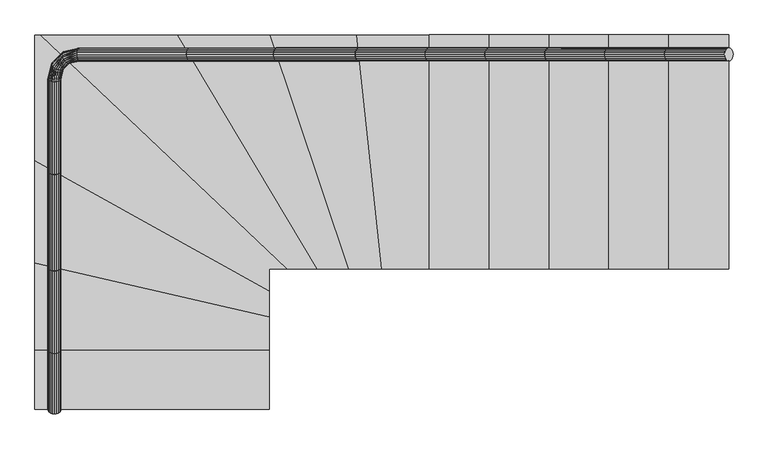
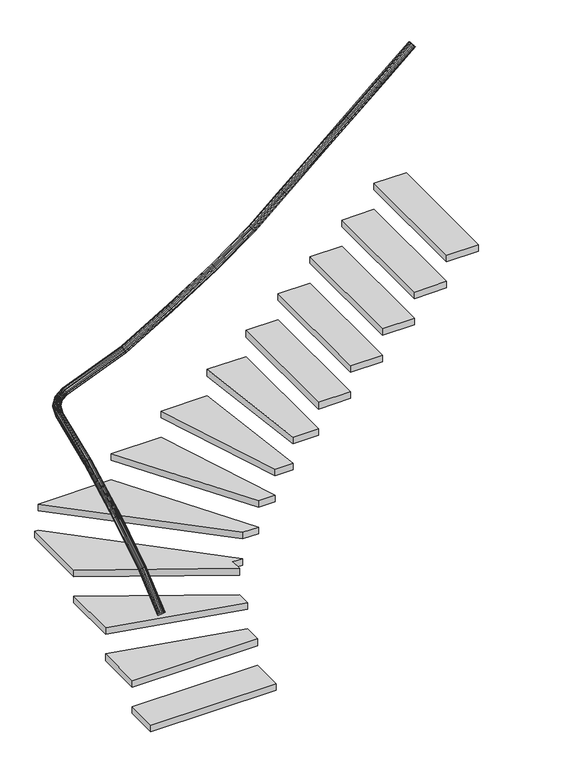
"""IFC4 building model written with IfcOpenShell, lengths in millimetres: stair geometry, 0_3d_modell."""

import ifcopenshell
import ifcopenshell.guid

model = None  # the IFC model being written
_history = None  # IfcOwnerHistory: only IFC2X3 demands one
_inside = {}  # id of a spatial element -> (the spatial element, [elements in it])
_under = {}  # id of a project, library or spatial element -> (it, [spatial elements below it])
_declared = {}  # id of a project -> (the project, [libraries it declares])
_typed = {}  # id of a type object -> (the type object, [elements of that type])
_made_of = {}  # id of a material, layer set ... -> (it, [elements and type objects made of it])


def new_model(schema):
    """Start an empty IFC model of exactly this schema.

    Asked for "IFC4X3", IfcOpenShell would pick the latest addendum, in which some entities
    have other attributes; the version numbers below select the first issue.
    IFC2X3 requires an IfcOwnerHistory on every rooted entity: one is made here for all.
    """
    global model, _history
    if schema == "IFC4X3":
        model = ifcopenshell.file(schema_version=(4, 3, 0, 0))
    else:
        model = ifcopenshell.file(schema=schema)
    _inside.clear()
    _under.clear()
    _declared.clear()
    _typed.clear()
    _made_of.clear()
    _history = None
    if model.schema == "IFC2X3":
        org = make("IfcOrganization", Name="unknown")
        user = make(
            "IfcPersonAndOrganization",
            ThePerson=make("IfcPerson", FamilyName="unknown"),
            TheOrganization=org,
        )
        app = make(
            "IfcApplication",
            ApplicationDeveloper=org,
            Version="unknown",
            ApplicationFullName="unknown",
            ApplicationIdentifier="unknown",
        )
        _history = make(
            "IfcOwnerHistory",
            OwningUser=user,
            OwningApplication=app,
            ChangeAction="ADDED",
            CreationDate=0,
        )
    return model


def make(cls, **values):
    """One entity of the class cls with the attributes given. An attribute that is None is left unset."""
    return model.create_entity(
        cls, **{name: value for name, value in values.items() if value is not None}
    )


def rooted(cls, **values):
    """An entity with a GlobalId (a new one), such as an element, a storey or a relation."""
    return make(cls, GlobalId=ifcopenshell.guid.new(), OwnerHistory=_history, **values)


def si_unit(unit_type, name, prefix=None):
    """IfcSIUnit, for example si_unit("LENGTHUNIT", "METRE", prefix="MILLI")."""
    return make("IfcSIUnit", UnitType=unit_type, Prefix=prefix, Name=name)


def assignment(units):
    """IfcUnitAssignment: the units of a project."""
    return None if units is None else make("IfcUnitAssignment", Units=units)


def point(xyz):
    """IfcCartesianPoint."""
    return None if xyz is None else make("IfcCartesianPoint", Coordinates=xyz)


def direction(xyz):
    """IfcDirection."""
    return None if xyz is None else make("IfcDirection", DirectionRatios=xyz)


def frame(location, z_axis=None, x_axis=None):
    """IfcAxis2Placement3D, a coordinate frame: its origin and axes. An axis left out is left unset."""
    return make(
        "IfcAxis2Placement3D",
        Location=point(location),
        Axis=direction(z_axis),
        RefDirection=direction(x_axis),
    )


def origin():
    """The frame at (0, 0, 0) with its axes left unset."""
    return frame((0.0, 0.0, 0.0))


def origin_with_axes():
    """The frame at (0, 0, 0) with the z axis (0, 0, 1) and the x axis (1, 0, 0) written out."""
    return frame((0.0, 0.0, 0.0), z_axis=(0.0, 0.0, 1.0), x_axis=(1.0, 0.0, 0.0))


def place(relative_to, where):
    """IfcLocalPlacement: puts the frame where relative to a parent placement (None: the world)."""
    return make(
        "IfcLocalPlacement", PlacementRelTo=relative_to, RelativePlacement=where
    )


def context(
    kind, dimensions, precision=None, world=None, true_north=None, identifier=None
):
    """IfcGeometricRepresentationContext, for example the 3D "Model" context."""
    return make(
        "IfcGeometricRepresentationContext",
        ContextIdentifier=identifier,
        ContextType=kind,
        CoordinateSpaceDimension=dimensions,
        Precision=precision,
        WorldCoordinateSystem=world,
        TrueNorth=true_north,
    )


def project(units=None, contexts=None):
    """IfcProject with its units and contexts."""
    return rooted(
        "IfcProject",
        Name="project",
        RepresentationContexts=contexts,
        UnitsInContext=assignment(units),
    )


def spatial(cls, under=None, at=None, **own):
    """A site, building, storey or space (cls), placed at a placement, below another one or the project."""
    s = rooted(cls, ObjectPlacement=at, **own)
    if under is not None:
        _under.setdefault(under.id(), (under, []))[1].append(s)
    return s


def polyline(points):
    """IfcPolyline through the points."""
    return make("IfcPolyline", Points=[point(p) for p in points])


def outline(outer, holes=None, kind="AREA"):
    """IfcArbitraryClosedProfileDef: a profile drawn as a closed curve; with holes, ...WithVoids."""
    if holes is None:
        return make("IfcArbitraryClosedProfileDef", ProfileType=kind, OuterCurve=outer)
    return make(
        "IfcArbitraryProfileDefWithVoids",
        ProfileType=kind,
        OuterCurve=outer,
        InnerCurves=holes,
    )


def extrude(swept, where, along, depth):
    """IfcExtrudedAreaSolid: the profile swept, set in the frame where, extruded along a direction by depth."""
    return make(
        "IfcExtrudedAreaSolid",
        SweptArea=swept,
        Position=where,
        ExtrudedDirection=direction(along),
        Depth=depth,
    )


def faces_of(points, faces, orient=None, outer=None):
    """IfcFace entities. A face is a list of loops; a loop is a list of indices into points, from 0.

    orient and outer hold one flag for each loop. By default every Orientation is true, the
    first loop of a face is its IfcFaceOuterBound and the others are IfcFaceBound.
    """
    made = []
    for i, loops in enumerate(faces):
        bounds = []
        for j, loop in enumerate(loops):
            is_outer = j == 0 if outer is None else outer[i][j]
            bounds.append(
                make(
                    "IfcFaceOuterBound" if is_outer else "IfcFaceBound",
                    Bound=make("IfcPolyLoop", Polygon=[points[k] for k in loop]),
                    Orientation=True if orient is None else orient[i][j],
                )
            )
        made.append(make("IfcFace", Bounds=bounds))
    return made


def faceted_brep(points, faces, orient=None, outer=None, voids=None):
    """IfcFacetedBrep: a solid bounded by flat faces; with voids (closed shells), ...WithVoids."""
    shared = [point(p) for p in points]
    hull = make("IfcClosedShell", CfsFaces=faces_of(shared, faces, orient, outer))
    if voids is None:
        return make("IfcFacetedBrep", Outer=hull)
    return make(
        "IfcFacetedBrepWithVoids",
        Outer=hull,
        Voids=[
            make(cls, CfsFaces=faces_of(shared, fs, o, b)) for cls, fs, o, b in voids
        ],
    )


def shape(context_of_items, identifier, shape_type, items):
    """IfcShapeRepresentation: the items that make up one representation, for example the "Body"."""
    return make(
        "IfcShapeRepresentation",
        ContextOfItems=context_of_items,
        RepresentationIdentifier=identifier,
        RepresentationType=shape_type,
        Items=items,
    )


def source(mapping_origin, context_of_items, identifier, shape_type, items):
    """IfcRepresentationMap: a shape defined once, which mapped items show again and again."""
    return make(
        "IfcRepresentationMap",
        MappingOrigin=mapping_origin,
        MappedRepresentation=shape(context_of_items, identifier, shape_type, items),
    )


def transform(
    local_origin,
    x_axis=None,
    y_axis=None,
    z_axis=None,
    scale=None,
    scale2=None,
    scale3=None,
    uniform=True,
):
    """IfcCartesianTransformationOperator3D, or its non-uniform kind. x_axis, y_axis, z_axis: its Axis1, 2, 3."""
    if uniform:
        return make(
            "IfcCartesianTransformationOperator3D",
            Axis1=direction(x_axis),
            Axis2=direction(y_axis),
            LocalOrigin=point(local_origin),
            Scale=scale,
            Axis3=direction(z_axis),
        )
    return make(
        "IfcCartesianTransformationOperator3DnonUniform",
        Axis1=direction(x_axis),
        Axis2=direction(y_axis),
        LocalOrigin=point(local_origin),
        Scale=scale,
        Axis3=direction(z_axis),
        Scale2=scale2,
        Scale3=scale3,
    )


def mapped(mapping_source, mapping_target):
    """IfcMappedItem: shows the shape of a source again, moved by a transform."""
    return make(
        "IfcMappedItem", MappingSource=mapping_source, MappingTarget=mapping_target
    )


def made_of(thing, what):
    """Note that an element or type object is made of a material, layer set ...; save() writes the relation."""
    if what is not None:
        _made_of.setdefault(what.id(), (what, []))[1].append(thing)
    return thing


def element(
    cls,
    number,
    at=None,
    inside=None,
    cuts=None,
    type_object=None,
    material=None,
    context=None,
    identifier="Body",
    shape_type=None,
    held_by="IfcProductDefinitionShape",
    body=None,
    shapes=None,
    **own,
):
    """One element of the class cls, such as IfcWall. Its Tag is "e" and its number.

    at: its placement. inside: the storey or other place that contains it. cuts: it is an
    opening in that element (IfcRelVoidsElement). A single representation is given by context,
    identifier, shape_type and body (its items); several are given by shapes. held_by: the class
    of the entity that holds the representations. save() writes the other relations.
    """
    e = rooted(cls, Tag="e%d" % number, ObjectPlacement=at, **own)
    if body is not None:
        shapes = [shape(context, identifier, shape_type, body)]
    if shapes is not None:
        e.Representation = make(held_by, Representations=shapes)
    if inside is not None:
        _inside.setdefault(inside.id(), (inside, []))[1].append(e)
    if cuts is not None:
        rooted(
            "IfcRelVoidsElement", RelatingBuildingElement=cuts, RelatedOpeningElement=e
        )
    if type_object is not None:
        _typed.setdefault(type_object.id(), (type_object, []))[1].append(e)
    return made_of(e, material)


def aggregate(whole, parts):
    """IfcRelAggregates: a whole, such as a stair, and the parts it consists of."""
    return rooted("IfcRelAggregates", RelatingObject=whole, RelatedObjects=parts)


def save(model, path):
    """Write the relations noted so far, then the file.

    IfcRelAggregates (storeys below a building ...), IfcRelContainedInSpatialStructure (elements
    in a storey), IfcRelDefinesByType, IfcRelAssociatesMaterial and IfcRelDeclares: one each for
    every whole, place, type object, material and project.
    """
    for whole, parts in _under.values():
        aggregate(whole, parts)
    for where, things in _inside.values():
        rooted(
            "IfcRelContainedInSpatialStructure",
            RelatedElements=things,
            RelatingStructure=where,
        )
    for kind, things in _typed.values():
        rooted("IfcRelDefinesByType", RelatedObjects=things, RelatingType=kind)
    for what, things in _made_of.values():
        rooted("IfcRelAssociatesMaterial", RelatedObjects=things, RelatingMaterial=what)
    for by, libraries in _declared.values():
        rooted("IfcRelDeclares", RelatingContext=by, RelatedDefinitions=libraries)
    model.write(path)


def stair_7a128c32(model_context):
    return source(origin(), model_context, "Body", "SolidModel", [
        faceted_brep([(51.2235871, 11.6788974, 875.6088541), (50.0, 16.9018591, 869.5592366), (51.2235871, 22.1248208, 863.5096191), (54.7745751, 26.8365226, 858.0521803), (60.3053687, 30.5757504, 853.7211323), (67.2745751, 32.9764824, 850.9404284), (75.0, 33.8037182, 849.9822631), (82.7254249, 32.9764824, 850.9404284), (89.6946313, 30.5757504, 853.7211323), (95.2254249, 26.8365226, 858.0521803), (98.7764129, 22.1248208, 863.5096191), (100.0, 16.9018591, 869.5592366), (98.7764129, 11.6788974, 875.6088541), (95.2254249, 6.9671956, 881.0662929), (89.6946313, 3.2279679, 885.3973409), (82.7254249, 0.8272359, 888.1780448), (75.0, 0.0, 889.1362101), (67.2745751, 0.8272359, 888.1780448), (60.3053687, 3.2279679, 885.3973409), (54.7745751, 6.9671956, 881.0662929), (51.2235871, 251.6675536, 1061.6862641), (50.0, 246.9018591, 1068.1306652), (51.2235871, 242.1361647, 1074.5750662), (54.7745751, 237.8369696, 1080.3886444), (60.3053687, 234.4251091, 1085.0023262), (67.2745751, 232.2345598, 1087.9644922), (75.0, 231.4797479, 1088.985185), (82.7254249, 232.2345598, 1087.9644922), (89.6946313, 234.4251091, 1085.0023262), (95.2254249, 237.8369696, 1080.3886444), (98.7764129, 242.1361647, 1074.5750662), (100.0, 246.9018591, 1068.1306652), (98.7764129, 251.6675536, 1061.6862641), (95.2254249, 255.9667486, 1055.872686), (89.6946313, 259.3786091, 1051.2590042), (82.7254249, 261.5691584, 1048.2968382), (75.0, 262.3239703, 1047.2761453), (67.2745751, 261.5691584, 1048.2968382), (60.3053687, 259.3786091, 1051.2590042), (54.7745751, 255.9667486, 1055.872686)], [[[0, 1, 2, 3, 4, 5, 6, 7, 8, 9, 10, 11, 12, 13, 14, 15, 16, 17, 18, 19]], [[20, 21, 22, 23, 24, 25, 26, 27, 28, 29, 30, 31, 32, 33, 34, 35, 36, 37, 38, 39]], [[21, 1, 0, 22]], [[22, 0, 19, 23]], [[23, 19, 18, 24]], [[24, 18, 17, 25]], [[25, 17, 16, 26]], [[26, 16, 15, 27]], [[27, 15, 14, 28]], [[28, 14, 13, 29]], [[29, 13, 12, 30]], [[30, 12, 11, 31]], [[31, 11, 10, 32]], [[32, 10, 9, 33]], [[33, 9, 8, 34]], [[34, 8, 7, 35]], [[35, 7, 6, 36]], [[36, 6, 5, 37]], [[37, 5, 4, 38]], [[38, 4, 3, 39]], [[39, 3, 2, 20]], [[20, 2, 1, 21]]]),
        extrude(outline(polyline([(900.0, 373.9346688), (0.0, 579.8690495), (0.0, 973.1970565), (900.0, 473.824936), (900.0, 373.9346688)])), frame((0.0, 0.0, 397.1428571), z_axis=(0.0, 0.0, 1.0), x_axis=(1.0, 0.0, 0.0)), (0.0, 0.0, 1.0), 50.0),
        extrude(outline(polyline([(1.2235871, -7.9923214), (0.0, 0.0), (1.2235871, 7.9923214), (4.7745751, 15.2022986), (10.3053687, 20.924169), (17.2745751, 24.5978359), (25.0, 25.8636953), (32.7254248, 24.5978359), (39.6946313, 20.924169), (45.2254248, 15.2022986), (48.7764129, 7.9923214), (50.0, 0.0), (48.7764129, -7.9923214), (45.2254248, -15.2022987), (39.6946313, -20.9241691), (32.7254248, -24.597836), (25.0, -25.8636953), (17.2745751, -24.597836), (10.3053687, -20.9241691), (4.7745751, -15.2022987), (1.2235871, -7.9923214)])), frame((1744.6018366, 1406.9018591, 2656.7020937), z_axis=(0.7569287102857354, 0.0, 0.6534974579485168), x_axis=(0.0, -1.0, 0.0)), (0.0, 0.0, 1.0), 303.8595272),
        faceted_brep([(1509.6138519, 1405.678272, 2464.383151), (1514.6018366, 1406.9018591, 2458.1306652), (1519.5898213, 1405.678272, 2451.8781793), (1524.0895473, 1402.127284, 2446.2377304), (1527.6605501, 1396.5964904, 2441.7614447), (1529.9532751, 1389.627284, 2438.8874925), (1530.7432942, 1381.9018591, 2437.897196), (1529.9532751, 1374.1764343, 2438.8874925), (1527.6605501, 1367.2072278, 2441.7614447), (1524.0895473, 1361.6764343, 2446.2377304), (1519.5898213, 1358.1254462, 2451.8781793), (1514.6018366, 1356.9018591, 2458.1306652), (1509.6138519, 1358.1254462, 2464.383151), (1505.1141259, 1361.6764343, 2470.0236), (1501.5431231, 1367.2072278, 2474.4998856), (1499.2503981, 1374.1764343, 2477.3738379), (1498.460379, 1381.9018591, 2478.3641344), (1499.2503981, 1389.627284, 2477.3738379), (1501.5431231, 1396.5964904, 2474.4998856), (1505.1141259, 1402.127284, 2470.0236), (1749.8247983, 1405.678272, 2650.6524762), (1744.6018366, 1406.9018591, 2656.7020937), (1739.3788749, 1405.678272, 2662.7517113), (1734.6671731, 1402.127284, 2668.2091501), (1730.9279453, 1396.5964904, 2672.540198), (1728.5272134, 1389.627284, 2675.320902), (1727.6999775, 1381.9018591, 2676.2790673), (1728.5272134, 1374.1764343, 2675.320902), (1730.9279453, 1367.2072278, 2672.540198), (1734.6671731, 1361.6764343, 2668.2091501), (1739.3788749, 1358.1254462, 2662.7517113), (1744.6018366, 1356.9018591, 2656.7020937), (1749.8247983, 1358.1254462, 2650.6524762), (1754.5365001, 1361.6764343, 2645.1950374), (1758.2757279, 1367.2072278, 2640.8639895), (1760.6764598, 1374.1764343, 2638.0832855), (1761.5036957, 1381.9018591, 2637.1251202), (1760.6764598, 1389.627284, 2638.0832855), (1758.2757279, 1396.5964904, 2640.8639895), (1754.5365001, 1402.127284, 2645.1950374)], [[[0, 1, 2, 3, 4, 5, 6, 7, 8, 9, 10, 11, 12, 13, 14, 15, 16, 17, 18, 19]], [[20, 21, 22, 23, 24, 25, 26, 27, 28, 29, 30, 31, 32, 33, 34, 35, 36, 37, 38, 39]], [[21, 1, 0, 22]], [[22, 0, 19, 23]], [[23, 19, 18, 24]], [[24, 18, 17, 25]], [[25, 17, 16, 26]], [[26, 16, 15, 27]], [[27, 15, 14, 28]], [[28, 14, 13, 29]], [[29, 13, 12, 30]], [[30, 12, 11, 31]], [[31, 11, 10, 32]], [[32, 10, 9, 33]], [[33, 9, 8, 34]], [[34, 8, 7, 35]], [[35, 7, 6, 36]], [[36, 6, 5, 37]], [[37, 5, 4, 38]], [[38, 4, 3, 39]], [[39, 3, 2, 20]], [[20, 2, 1, 21]]]),
        faceted_brep([(51.2235871, 242.1361647, 1074.5750662), (50.0, 246.9018591, 1068.1306652), (51.2235871, 251.6675536, 1061.6862641), (54.7745751, 255.9667486, 1055.872686), (60.3053687, 259.3786091, 1051.2590042), (67.2745751, 261.5691584, 1048.2968382), (75.0, 262.3239703, 1047.2761453), (82.7254249, 261.5691584, 1048.2968382), (89.6946313, 259.3786091, 1051.2590042), (95.2254249, 255.9667486, 1055.872686), (98.7764129, 251.6675536, 1061.6862641), (100.0, 246.9018591, 1068.1306652), (98.7764129, 242.1361647, 1074.5750662), (95.2254249, 237.8369696, 1080.3886444), (89.6946313, 234.4251091, 1085.0023262), (82.7254249, 232.2345598, 1087.9644922), (75.0, 231.4797479, 1088.985185), (67.2745751, 232.2345598, 1087.9644922), (60.3053687, 234.4251091, 1085.0023262), (54.7745751, 237.8369696, 1080.3886444), (51.2235871, 566.7337566, 1259.7925307), (50.0, 562.7078511, 1266.7020937), (51.2235871, 558.6819455, 1273.6116568), (54.7745751, 555.0501237, 1279.8448636), (60.3053687, 552.1678935, 1284.7915646), (67.2745751, 550.3173878, 1287.9675421), (75.0, 549.679747, 1289.0619094), (82.7254249, 550.3173878, 1287.9675421), (89.6946313, 552.1678935, 1284.7915646), (95.2254249, 555.0501237, 1279.8448636), (98.7764129, 558.6819455, 1273.6116568), (100.0, 562.7078511, 1266.7020937), (98.7764129, 566.7337566, 1259.7925307), (95.2254249, 570.3655785, 1253.5593239), (89.6946313, 573.2478087, 1248.6126229), (82.7254249, 575.0983143, 1245.4366454), (75.0, 575.7359551, 1244.3422781), (67.2745751, 575.0983143, 1245.4366454), (60.3053687, 573.2478087, 1248.6126229), (54.7745751, 570.3655785, 1253.5593239)], [[[0, 1, 2, 3, 4, 5, 6, 7, 8, 9, 10, 11, 12, 13, 14, 15, 16, 17, 18, 19]], [[20, 21, 22, 23, 24, 25, 26, 27, 28, 29, 30, 31, 32, 33, 34, 35, 36, 37, 38, 39]], [[21, 1, 0, 22]], [[22, 0, 19, 23]], [[23, 19, 18, 24]], [[24, 18, 17, 25]], [[25, 17, 16, 26]], [[26, 16, 15, 27]], [[27, 15, 14, 28]], [[28, 14, 13, 29]], [[29, 13, 12, 30]], [[30, 12, 11, 31]], [[31, 11, 10, 32]], [[32, 10, 9, 33]], [[33, 9, 8, 34]], [[34, 8, 7, 35]], [[35, 7, 6, 36]], [[36, 6, 5, 37]], [[37, 5, 4, 38]], [[38, 4, 3, 39]], [[39, 3, 2, 20]], [[20, 2, 1, 21]]]),
        extrude(outline(polyline([(1.2235871, -7.9923214), (0.0, 0.0), (1.2235871, 7.9923214), (4.7745751, 15.2022986), (10.3053687, 20.9241691), (17.2745751, 24.597836), (25.0, 25.8636953), (32.7254248, 24.597836), (39.6946313, 20.9241691), (45.2254248, 15.2022986), (48.7764129, 7.9923214), (50.0, 0.0), (48.7764129, -7.9923214), (45.2254248, -15.2022986), (39.6946313, -20.924169), (32.7254248, -24.5978359), (25.0, -25.8636953), (17.2745751, -24.5978359), (10.3053687, -20.924169), (4.7745751, -15.2022986), (1.2235871, -7.9923214)])), frame((2434.6018366, 1406.9018591, 3252.4163795), z_axis=(0.7569287102857536, 0.0, 0.6534974579484957), x_axis=(0.0, -1.0, 0.0)), (0.0, 0.0, 1.0), 303.8595272),
        faceted_brep([(925.538539, 1405.678272, 2067.8109967), (929.7020117, 1406.9018591, 2060.987808), (933.8654844, 1405.678272, 2054.1646194), (937.6214074, 1402.127284, 2048.009332), (940.6021247, 1396.5964904, 2043.1244683), (942.515863, 1389.627284, 2039.9881928), (943.1752923, 1381.9018591, 2038.9075058), (942.515863, 1374.1764343, 2039.9881928), (940.6021247, 1367.2072278, 2043.1244683), (937.6214074, 1361.6764343, 2048.009332), (933.8654844, 1358.1254462, 2054.1646194), (929.7020117, 1356.9018591, 2060.987808), (925.538539, 1358.1254462, 2067.8109967), (921.782616, 1361.6764343, 2073.966284), (918.8018987, 1367.2072278, 2078.8511477), (916.8881603, 1374.1764343, 2081.9874233), (916.228731, 1381.9018591, 2083.0681102), (916.8881603, 1389.627284, 2081.9874233), (918.8018987, 1396.5964904, 2078.8511477), (921.782616, 1402.127284, 2073.966284), (1249.3489942, 1405.678272, 2252.9513864), (1244.8437697, 1406.9018591, 2259.5592366), (1240.3385453, 1405.678272, 2266.1670868), (1236.2743236, 1402.127284, 2272.1281145), (1233.048939, 1396.5964904, 2276.858813), (1230.9781146, 1389.627284, 2279.8961083), (1230.2645572, 1381.9018591, 2280.942689), (1230.9781146, 1374.1764343, 2279.8961083), (1233.048939, 1367.2072278, 2276.858813), (1236.2743236, 1361.6764343, 2272.1281145), (1240.3385453, 1358.1254462, 2266.1670868), (1244.8437697, 1356.9018591, 2259.5592366), (1249.3489942, 1358.1254462, 2252.9513864), (1253.4132159, 1361.6764343, 2246.9903587), (1256.6386004, 1367.2072278, 2242.2596602), (1258.7094248, 1374.1764343, 2239.2223649), (1259.4229823, 1381.9018591, 2238.1757842), (1258.7094248, 1389.627284, 2239.2223649), (1256.6386004, 1396.5964904, 2242.2596602), (1253.4132159, 1402.127284, 2246.9903587)], [[[0, 1, 2, 3, 4, 5, 6, 7, 8, 9, 10, 11, 12, 13, 14, 15, 16, 17, 18, 19]], [[20, 21, 22, 23, 24, 25, 26, 27, 28, 29, 30, 31, 32, 33, 34, 35, 36, 37, 38, 39]], [[21, 1, 0, 22]], [[22, 0, 19, 23]], [[23, 19, 18, 24]], [[24, 18, 17, 25]], [[25, 17, 16, 26]], [[26, 16, 15, 27]], [[27, 15, 14, 28]], [[28, 14, 13, 29]], [[29, 13, 12, 30]], [[30, 12, 11, 31]], [[31, 11, 10, 32]], [[32, 10, 9, 33]], [[33, 9, 8, 34]], [[34, 8, 7, 35]], [[35, 7, 6, 36]], [[36, 6, 5, 37]], [[37, 5, 4, 38]], [[38, 4, 3, 39]], [[39, 3, 2, 20]], [[20, 2, 1, 21]]]),
        extrude(outline(polyline([(900.0, 473.824936), (0.0, 973.1970565), (0.0, 1456.9018591), (22.6704161, 1456.9018591), (970.0, 556.9018591), (900.0, 556.9018591), (900.0, 473.824936)])), frame((0.0, 0.0, 595.7142857), z_axis=(0.0, 0.0, 1.0), x_axis=(1.0, 0.0, 0.0)), (0.0, 0.0, 1.0), 50.0),
        faceted_brep([(1240.3385453, 1405.678272, 2266.1670868), (1244.8437697, 1406.9018591, 2259.5592366), (1249.3489942, 1405.678272, 2252.9513864), (1253.4132159, 1402.127284, 2246.9903587), (1256.6386004, 1396.5964904, 2242.2596602), (1258.7094248, 1389.627284, 2239.2223649), (1259.4229823, 1381.9018591, 2238.1757842), (1258.7094248, 1374.1764343, 2239.2223649), (1256.6386004, 1367.2072278, 2242.2596602), (1253.4132159, 1361.6764343, 2246.9903587), (1249.3489942, 1358.1254462, 2252.9513864), (1244.8437697, 1356.9018591, 2259.5592366), (1240.3385453, 1358.1254462, 2266.1670868), (1236.2743236, 1361.6764343, 2272.1281145), (1233.048939, 1367.2072278, 2276.858813), (1230.9781146, 1374.1764343, 2279.8961083), (1230.2645572, 1381.9018591, 2280.942689), (1230.9781146, 1389.627284, 2279.8961083), (1233.048939, 1396.5964904, 2276.858813), (1236.2743236, 1402.127284, 2272.1281145), (1519.5898213, 1405.678272, 2451.8781793), (1514.6018366, 1406.9018591, 2458.1306652), (1509.6138519, 1405.678272, 2464.383151), (1505.1141259, 1402.127284, 2470.0236), (1501.5431231, 1396.5964904, 2474.4998856), (1499.2503981, 1389.627284, 2477.3738379), (1498.460379, 1381.9018591, 2478.3641344), (1499.2503981, 1374.1764343, 2477.3738379), (1501.5431231, 1367.2072278, 2474.4998856), (1505.1141259, 1361.6764343, 2470.0236), (1509.6138519, 1358.1254462, 2464.383151), (1514.6018366, 1356.9018591, 2458.1306652), (1519.5898213, 1358.1254462, 2451.8781793), (1524.0895473, 1361.6764343, 2446.2377304), (1527.6605501, 1367.2072278, 2441.7614447), (1529.9532751, 1374.1764343, 2438.8874925), (1530.7432942, 1381.9018591, 2437.897196), (1529.9532751, 1389.627284, 2438.8874925), (1527.6605501, 1396.5964904, 2441.7614447), (1524.0895473, 1402.127284, 2446.2377304)], [[[0, 1, 2, 3, 4, 5, 6, 7, 8, 9, 10, 11, 12, 13, 14, 15, 16, 17, 18, 19]], [[20, 21, 22, 23, 24, 25, 26, 27, 28, 29, 30, 31, 32, 33, 34, 35, 36, 37, 38, 39]], [[21, 1, 0, 22]], [[22, 0, 19, 23]], [[23, 19, 18, 24]], [[24, 18, 17, 25]], [[25, 17, 16, 26]], [[26, 16, 15, 27]], [[27, 15, 14, 28]], [[28, 14, 13, 29]], [[29, 13, 12, 30]], [[30, 12, 11, 31]], [[31, 11, 10, 32]], [[32, 10, 9, 33]], [[33, 9, 8, 34]], [[34, 8, 7, 35]], [[35, 7, 6, 36]], [[36, 6, 5, 37]], [[37, 5, 4, 38]], [[38, 4, 3, 39]], [[39, 3, 2, 20]], [[20, 2, 1, 21]]]),
        extrude(outline(polyline([(1204.4816265, 556.9018591), (904.7220467, 1456.9018591), (1236.8921564, 1456.9018591), (1332.3115168, 556.9018591), (1204.4816265, 556.9018591)])), frame((0.0, 0.0, 1191.4285714), z_axis=(0.0, 0.0, 1.0), x_axis=(1.0, 0.0, 0.0)), (0.0, 0.0, 1.0), 50.0),
        extrude(outline(polyline([(900.0, 16.9018591), (0.0, 16.9018591), (0.0, 246.9018591), (900.0, 246.9018591), (900.0, 16.9018591)])), origin_with_axes(), (0.0, 0.0, 1.0), 50.0),
        faceted_brep([(589.9532071, 1405.678272, 1869.6030507), (593.5012683, 1406.9018591, 1862.4163795), (597.0493296, 1405.678272, 1855.2297082), (600.2500819, 1402.127284, 1848.7465184), (602.7902133, 1396.5964904, 1843.6014299), (604.421078, 1389.627284, 1840.2980797), (604.9830357, 1381.9018591, 1839.1598228), (604.421078, 1374.1764343, 1840.2980797), (602.7902133, 1367.2072278, 1843.6014299), (600.2500819, 1361.6764343, 1848.7465184), (597.0493296, 1358.1254462, 1855.2297082), (593.5012683, 1356.9018591, 1862.4163795), (589.9532071, 1358.1254462, 1869.6030507), (586.7524548, 1361.6764343, 1876.0862405), (584.2123234, 1367.2072278, 1881.231329), (582.5814586, 1374.1764343, 1884.5346792), (582.019501, 1381.9018591, 1885.6729361), (582.5814586, 1389.627284, 1884.5346792), (584.2123234, 1396.5964904, 1881.231329), (586.7524548, 1402.127284, 1876.0862405), (933.8654844, 1405.678272, 2054.1646194), (929.7020117, 1406.9018591, 2060.987808), (925.538539, 1405.678272, 2067.8109967), (921.782616, 1402.127284, 2073.966284), (918.8018987, 1396.5964904, 2078.8511477), (916.8881603, 1389.627284, 2081.9874233), (916.228731, 1381.9018591, 2083.0681102), (916.8881603, 1374.1764343, 2081.9874233), (918.8018987, 1367.2072278, 2078.8511477), (921.782616, 1361.6764343, 2073.966284), (925.538539, 1358.1254462, 2067.8109967), (929.7020117, 1356.9018591, 2060.987808), (933.8654844, 1358.1254462, 2054.1646194), (937.6214074, 1361.6764343, 2048.009332), (940.6021247, 1367.2072278, 2043.1244683), (942.515863, 1374.1764343, 2039.9881928), (943.1752923, 1381.9018591, 2038.9075058), (942.515863, 1389.627284, 2039.9881928), (940.6021247, 1396.5964904, 2043.1244683), (937.6214074, 1402.127284, 2048.009332)], [[[0, 1, 2, 3, 4, 5, 6, 7, 8, 9, 10, 11, 12, 13, 14, 15, 16, 17, 18, 19]], [[20, 21, 22, 23, 24, 25, 26, 27, 28, 29, 30, 31, 32, 33, 34, 35, 36, 37, 38, 39]], [[21, 1, 0, 22]], [[22, 0, 19, 23]], [[23, 19, 18, 24]], [[24, 18, 17, 25]], [[25, 17, 16, 26]], [[26, 16, 15, 27]], [[27, 15, 14, 28]], [[28, 14, 13, 29]], [[29, 13, 12, 30]], [[30, 12, 11, 31]], [[31, 11, 10, 32]], [[32, 10, 9, 33]], [[33, 9, 8, 34]], [[34, 8, 7, 35]], [[35, 7, 6, 36]], [[36, 6, 5, 37]], [[37, 5, 4, 38]], [[38, 4, 3, 39]], [[39, 3, 2, 20]], [[20, 2, 1, 21]]]),
        extrude(outline(polyline([(1332.3115168, 556.9018591), (1236.8921564, 1456.9018591), (1514.6018366, 1456.9018591), (1514.6018366, 556.9018591), (1332.3115168, 556.9018591)])), frame((0.0, 0.0, 1390.0), z_axis=(0.0, 0.0, 1.0), x_axis=(1.0, 0.0, 0.0)), (0.0, 0.0, 1.0), 50.0),
        extrude(outline(polyline([(1744.6018366, 556.9018591), (1744.6018366, 1456.9018591), (1974.6018366, 1456.9018591), (1974.6018366, 556.9018591), (1744.6018366, 556.9018591)])), frame((0.0, 0.0, 1787.1428571), z_axis=(0.0, 0.0, 1.0), x_axis=(1.0, 0.0, 0.0)), (0.0, 0.0, 1.0), 50.0),
        extrude(outline(polyline([(1974.6018366, 556.9018591), (1974.6018366, 1456.9018591), (2204.6018366, 1456.9018591), (2204.6018366, 556.9018591), (1974.6018366, 556.9018591)])), frame((0.0, 0.0, 1985.7142857), z_axis=(0.0, 0.0, 1.0), x_axis=(1.0, 0.0, 0.0)), (0.0, 0.0, 1.0), 50.0),
        faceted_brep([(51.2235871, 1283.3224302, 1620.3777918), (50.0, 1286.3944101, 1612.9994356), (51.2235871, 1289.46639, 1605.6210794), (54.7745751, 1292.2376632, 1598.9649681), (60.3053687, 1294.436958, 1593.6826483), (67.2745751, 1295.8489921, 1590.2911902), (75.0, 1296.335546, 1589.1225734), (82.7254249, 1295.8489921, 1590.2911902), (89.6946313, 1294.436958, 1593.6826483), (95.2254249, 1292.2376632, 1598.9649681), (98.7764129, 1289.46639, 1605.6210794), (100.0, 1286.3944101, 1612.9994356), (98.7764129, 1283.3224302, 1620.3777918), (95.2254249, 1280.5511571, 1627.0339031), (89.6946313, 1278.3518623, 1632.3162229), (82.7254249, 1276.9398281, 1635.707681), (75.0, 1276.4532743, 1636.8762979), (67.2745751, 1276.9398281, 1635.707681), (60.3053687, 1278.3518623, 1632.3162229), (54.7745751, 1280.5511571, 1627.0339031), (65.0056921, 1348.8501513, 1638.9123688), (64.1990579, 1344.8271855, 1645.879395), (65.6181519, 1340.0232633, 1652.1644401), (69.1240635, 1334.9086261, 1657.1522801), (74.3736094, 1329.9839302, 1660.3546705), (80.8529277, 1325.7312391, 1661.4581391), (87.9277774, 1322.5668359, 1660.3546705), (94.9056231, 1320.8004745, 1657.1522801), (101.1034244, 1320.6050585, 1652.1644401), (105.9144976, 1321.9997167, 1645.879395), (108.8679012, 1324.8479302, 1638.9123688), (109.6745354, 1328.870896, 1631.9453426), (108.2554414, 1333.6748181, 1625.6602975), (104.7495298, 1338.7894554, 1620.6724574), (99.4999839, 1343.7141513, 1617.470067), (93.0206656, 1347.9668423, 1616.3665985), (85.9458159, 1351.1312455, 1617.470067), (78.9679702, 1352.8976069, 1620.6724574), (72.7701688, 1353.0930229, 1625.6602975), (67.9590957, 1351.6983647, 1631.9453426), (108.2142101, 1391.9456089, 1666.2859781), (105.3846216, 1389.0124344, 1673.2691208), (104.0019016, 1384.2169558, 1679.5687049), (104.2014005, 1378.028588, 1684.5680831), (105.96359, 1371.0530916, 1687.7778814), (109.1159746, 1363.9732768, 1688.8839026), (113.3499769, 1357.4821652, 1687.7778814), (118.2511434, 1352.215152, 1684.5680831), (123.3397137, 1348.6878091, 1679.5687049), (128.1175831, 1347.2454175, 1673.2691208), (132.1170605, 1348.0291684, 1666.2859781), (134.946649, 1350.962343, 1659.3028354), (136.329369, 1355.7578216, 1653.0032514), (136.1298701, 1361.9461894, 1648.0038732), (134.3676806, 1368.9216857, 1644.7940748), (131.215296, 1376.0015006, 1643.6880537), (126.9812936, 1382.4926122, 1644.7940748), (122.0801271, 1387.7596254, 1648.0038732), (116.9915569, 1391.2869683, 1653.0032514), (112.2136875, 1392.7293599, 1659.3028354), (170.8141891, 1406.9018591, 1691.7803901), (167.8223333, 1405.678272, 1699.1915978), (165.1233413, 1402.127284, 1705.8773449), (162.981409, 1396.5964904, 1711.1831838), (161.6062039, 1389.627284, 1714.5897421), (161.1323405, 1381.9018591, 1715.7635621), (161.6062039, 1374.1764343, 1714.5897421), (162.981409, 1367.2072278, 1711.1831838), (165.1233413, 1361.6764343, 1705.8773449), (167.8223333, 1358.1254462, 1699.1915978), (170.8141891, 1356.9018591, 1691.7803901), (173.8060448, 1358.1254462, 1684.3691823), (176.5050369, 1361.6764343, 1677.6834352), (178.6469691, 1367.2072278, 1672.3775963), (180.0221742, 1374.1764343, 1668.971038), (180.4960376, 1381.9018591, 1667.797218), (180.0221742, 1389.627284, 1668.971038), (178.6469691, 1396.5964904, 1672.3775963), (176.5050369, 1402.127284, 1677.6834352), (173.8060448, 1405.678272, 1684.3691823), (597.0493296, 1405.678272, 1855.2297082), (593.5012683, 1406.9018591, 1862.4163795), (589.9532071, 1405.678272, 1869.6030507), (586.7524548, 1402.127284, 1876.0862405), (584.2123234, 1396.5964904, 1881.231329), (582.5814586, 1389.627284, 1884.5346792), (582.019501, 1381.9018591, 1885.6729361), (582.5814586, 1374.1764343, 1884.5346792), (584.2123234, 1367.2072278, 1881.231329), (586.7524548, 1361.6764343, 1876.0862405), (589.9532071, 1358.1254462, 1869.6030507), (593.5012683, 1356.9018591, 1862.4163795), (597.0493296, 1358.1254462, 1855.2297082), (600.2500819, 1361.6764343, 1848.7465184), (602.7902133, 1367.2072278, 1843.6014299), (604.421078, 1374.1764343, 1840.2980797), (604.9830357, 1381.9018591, 1839.1598228), (604.421078, 1389.627284, 1840.2980797), (602.7902133, 1396.5964904, 1843.6014299), (600.2500819, 1402.127284, 1848.7465184)], [[[0, 1, 2, 3, 4, 5, 6, 7, 8, 9, 10, 11, 12, 13, 14, 15, 16, 17, 18, 19]], [[20, 1, 0]], [[20, 0, 21]], [[21, 0, 19]], [[21, 19, 22]], [[22, 19, 18]], [[22, 18, 23]], [[23, 18, 17]], [[23, 17, 24]], [[24, 17, 16]], [[24, 16, 25]], [[25, 16, 15]], [[25, 15, 26]], [[26, 15, 14]], [[26, 14, 27]], [[27, 14, 13]], [[27, 13, 28]], [[28, 13, 12]], [[28, 12, 29]], [[29, 12, 11]], [[29, 11, 30]], [[30, 11, 10]], [[30, 10, 31]], [[31, 10, 9]], [[31, 9, 32]], [[32, 9, 8]], [[32, 8, 33]], [[33, 8, 7]], [[33, 7, 34]], [[34, 7, 6]], [[34, 6, 35]], [[35, 6, 5]], [[35, 5, 36]], [[36, 5, 4]], [[36, 4, 37]], [[37, 4, 3]], [[37, 3, 38]], [[38, 3, 2]], [[38, 2, 39]], [[39, 2, 1]], [[39, 1, 20]], [[40, 20, 21]], [[40, 21, 41]], [[41, 21, 22]], [[41, 22, 42]], [[42, 22, 23]], [[42, 23, 43]], [[43, 23, 24]], [[43, 24, 44]], [[44, 24, 25]], [[44, 25, 45]], [[45, 25, 26]], [[45, 26, 46]], [[46, 26, 27]], [[46, 27, 47]], [[47, 27, 28]], [[47, 28, 48]], [[48, 28, 29]], [[48, 29, 49]], [[49, 29, 30]], [[49, 30, 50]], [[50, 30, 31]], [[50, 31, 51]], [[51, 31, 32]], [[51, 32, 52]], [[52, 32, 33]], [[52, 33, 53]], [[53, 33, 34]], [[53, 34, 54]], [[54, 34, 35]], [[54, 35, 55]], [[55, 35, 36]], [[55, 36, 56]], [[56, 36, 37]], [[56, 37, 57]], [[57, 37, 38]], [[57, 38, 58]], [[58, 38, 39]], [[58, 39, 59]], [[59, 39, 20]], [[59, 20, 40]], [[60, 40, 41]], [[60, 41, 61]], [[61, 41, 42]], [[61, 42, 62]], [[62, 42, 43]], [[62, 43, 63]], [[63, 43, 44]], [[63, 44, 64]], [[64, 44, 45]], [[64, 45, 65]], [[65, 45, 46]], [[65, 46, 66]], [[66, 46, 47]], [[66, 47, 67]], [[67, 47, 48]], [[67, 48, 68]], [[68, 48, 49]], [[68, 49, 69]], [[69, 49, 50]], [[69, 50, 70]], [[70, 50, 51]], [[70, 51, 71]], [[71, 51, 52]], [[71, 52, 72]], [[72, 52, 53]], [[72, 53, 73]], [[73, 53, 54]], [[73, 54, 74]], [[74, 54, 55]], [[74, 55, 75]], [[75, 55, 56]], [[75, 56, 76]], [[76, 56, 57]], [[76, 57, 77]], [[77, 57, 58]], [[77, 58, 78]], [[78, 58, 59]], [[78, 59, 79]], [[79, 59, 40]], [[79, 40, 60]], [[80, 81, 82, 83, 84, 85, 86, 87, 88, 89, 90, 91, 92, 93, 94, 95, 96, 97, 98, 99]], [[81, 60, 61, 82]], [[82, 61, 62, 83]], [[83, 62, 63, 84]], [[84, 63, 64, 85]], [[85, 64, 65, 86]], [[86, 65, 66, 87]], [[87, 66, 67, 88]], [[88, 67, 68, 89]], [[89, 68, 69, 90]], [[90, 69, 70, 91]], [[91, 70, 71, 92]], [[92, 71, 72, 93]], [[93, 72, 73, 94]], [[94, 73, 74, 95]], [[95, 74, 75, 96]], [[96, 75, 76, 97]], [[97, 76, 77, 98]], [[98, 77, 78, 99]], [[99, 78, 79, 80]], [[80, 79, 60, 81]]]),
        faceted_brep([(51.2235871, 558.6819455, 1273.6116568), (50.0, 562.7078511, 1266.7020937), (51.2235871, 566.7337566, 1259.7925307), (54.7745751, 570.3655785, 1253.5593239), (60.3053687, 573.2478087, 1248.6126229), (67.2745751, 575.0983143, 1245.4366454), (75.0, 575.7359551, 1244.3422781), (82.7254249, 575.0983143, 1245.4366454), (89.6946313, 573.2478087, 1248.6126229), (95.2254249, 570.3655785, 1253.5593239), (98.7764129, 566.7337566, 1259.7925307), (100.0, 562.7078511, 1266.7020937), (98.7764129, 558.6819455, 1273.6116568), (95.2254249, 555.0501237, 1279.8448636), (89.6946313, 552.1678935, 1284.7915646), (82.7254249, 550.3173878, 1287.9675421), (75.0, 549.679747, 1289.0619094), (67.2745751, 550.3173878, 1287.9675421), (60.3053687, 552.1678935, 1284.7915646), (54.7745751, 555.0501237, 1279.8448636), (51.2235871, 935.0213576, 1458.0478269), (50.0, 931.5827131, 1465.2735223), (51.2235871, 928.1440687, 1472.4992177), (54.7745751, 925.0420228, 1479.0176117), (60.3053687, 922.5802252, 1484.1906384), (67.2745751, 920.9996538, 1487.511926), (75.0, 920.4550261, 1488.6563638), (82.7254249, 920.9996538, 1487.511926), (89.6946313, 922.5802252, 1484.1906384), (95.2254249, 925.0420228, 1479.0176117), (98.7764129, 928.1440687, 1472.4992177), (100.0, 931.5827131, 1465.2735223), (98.7764129, 935.0213576, 1458.0478269), (95.2254249, 938.1234035, 1451.529433), (89.6946313, 940.5852011, 1446.3564062), (82.7254249, 942.1657724, 1443.0351186), (75.0, 942.7104002, 1441.8906809), (67.2745751, 942.1657724, 1443.0351186), (60.3053687, 940.5852011, 1446.3564062), (54.7745751, 938.1234035, 1451.529433)], [[[0, 1, 2, 3, 4, 5, 6, 7, 8, 9, 10, 11, 12, 13, 14, 15, 16, 17, 18, 19]], [[20, 21, 22, 23, 24, 25, 26, 27, 28, 29, 30, 31, 32, 33, 34, 35, 36, 37, 38, 39]], [[21, 1, 0, 22]], [[22, 0, 19, 23]], [[23, 19, 18, 24]], [[24, 18, 17, 25]], [[25, 17, 16, 26]], [[26, 16, 15, 27]], [[27, 15, 14, 28]], [[28, 14, 13, 29]], [[29, 13, 12, 30]], [[30, 12, 11, 31]], [[31, 11, 10, 32]], [[32, 10, 9, 33]], [[33, 9, 8, 34]], [[34, 8, 7, 35]], [[35, 7, 6, 36]], [[36, 6, 5, 37]], [[37, 5, 4, 38]], [[38, 4, 3, 39]], [[39, 3, 2, 20]], [[20, 2, 1, 21]]]),
        extrude(outline(polyline([(1514.6018366, 556.9018591), (1514.6018366, 1456.9018591), (1744.6018366, 1456.9018591), (1744.6018366, 556.9018591), (1514.6018366, 556.9018591)])), frame((0.0, 0.0, 1588.5714286), z_axis=(0.0, 0.0, 1.0), x_axis=(1.0, 0.0, 0.0)), (0.0, 0.0, 1.0), 50.0),
        extrude(outline(polyline([(970.0, 556.9018591), (22.6704161, 1456.9018591), (548.8803485, 1456.9018591), (1084.3313864, 556.9018591), (970.0, 556.9018591)])), frame((0.0, 0.0, 794.2857143), z_axis=(0.0, 0.0, 1.0), x_axis=(1.0, 0.0, 0.0)), (0.0, 0.0, 1.0), 50.0),
        extrude(outline(polyline([(2204.6018366, 556.9018591), (2204.6018366, 1456.9018591), (2434.6018366, 1456.9018591), (2434.6018366, 556.9018591), (2204.6018366, 556.9018591)])), frame((0.0, 0.0, 2184.2857143), z_axis=(0.0, 0.0, 1.0), x_axis=(1.0, 0.0, 0.0)), (0.0, 0.0, 1.0), 50.0),
        faceted_brep([(51.2235871, 928.1440687, 1472.4992177), (50.0, 931.5827131, 1465.2735223), (51.2235871, 935.0213576, 1458.0478269), (54.7745751, 938.1234035, 1451.529433), (60.3053687, 940.5852011, 1446.3564062), (67.2745751, 942.1657724, 1443.0351186), (75.0, 942.7104002, 1441.8906809), (82.7254249, 942.1657724, 1443.0351186), (89.6946313, 940.5852011, 1446.3564062), (95.2254249, 938.1234035, 1451.529433), (98.7764129, 935.0213576, 1458.0478269), (100.0, 931.5827131, 1465.2735223), (98.7764129, 928.1440687, 1472.4992177), (95.2254249, 925.0420228, 1479.0176117), (89.6946313, 922.5802252, 1484.1906384), (82.7254249, 920.9996538, 1487.511926), (75.0, 920.4550261, 1488.6563638), (67.2745751, 920.9996538, 1487.511926), (60.3053687, 922.5802252, 1484.1906384), (54.7745751, 925.0420228, 1479.0176117), (51.2235871, 1289.46639, 1605.6210794), (50.0, 1286.3944101, 1612.9994356), (51.2235871, 1283.3224302, 1620.3777918), (54.7745751, 1280.5511571, 1627.0339031), (60.3053687, 1278.3518623, 1632.3162229), (67.2745751, 1276.9398281, 1635.707681), (75.0, 1276.4532743, 1636.8762979), (82.7254249, 1276.9398281, 1635.707681), (89.6946313, 1278.3518623, 1632.3162229), (95.2254249, 1280.5511571, 1627.0339031), (98.7764129, 1283.3224302, 1620.3777918), (100.0, 1286.3944101, 1612.9994356), (98.7764129, 1289.46639, 1605.6210794), (95.2254249, 1292.2376632, 1598.9649681), (89.6946313, 1294.436958, 1593.6826483), (82.7254249, 1295.8489921, 1590.2911902), (75.0, 1296.335546, 1589.1225734), (67.2745751, 1295.8489921, 1590.2911902), (60.3053687, 1294.436958, 1593.6826483), (54.7745751, 1292.2376632, 1598.9649681)], [[[0, 1, 2, 3, 4, 5, 6, 7, 8, 9, 10, 11, 12, 13, 14, 15, 16, 17, 18, 19]], [[20, 21, 22, 23, 24, 25, 26, 27, 28, 29, 30, 31, 32, 33, 34, 35, 36, 37, 38, 39]], [[21, 1, 0, 22]], [[22, 0, 19, 23]], [[23, 19, 18, 24]], [[24, 18, 17, 25]], [[25, 17, 16, 26]], [[26, 16, 15, 27]], [[27, 15, 14, 28]], [[28, 14, 13, 29]], [[29, 13, 12, 30]], [[30, 12, 11, 31]], [[31, 11, 10, 32]], [[32, 10, 9, 33]], [[33, 9, 8, 34]], [[34, 8, 7, 35]], [[35, 7, 6, 36]], [[36, 6, 5, 37]], [[37, 5, 4, 38]], [[38, 4, 3, 39]], [[39, 3, 2, 20]], [[20, 2, 1, 21]]]),
        extrude(outline(polyline([(2434.6018366, 556.9018591), (2434.6018366, 1456.9018591), (2664.6018366, 1456.9018591), (2664.6018366, 556.9018591), (2434.6018366, 556.9018591)])), frame((0.0, 0.0, 2382.8571429), z_axis=(0.0, 0.0, 1.0), x_axis=(1.0, 0.0, 0.0)), (0.0, 0.0, 1.0), 50.0),
        extrude(outline(polyline([(1084.3313864, 556.9018591), (548.8803485, 1456.9018591), (904.7220467, 1456.9018591), (1204.4816265, 556.9018591), (1084.3313864, 556.9018591)])), frame((0.0, 0.0, 992.8571429), z_axis=(0.0, 0.0, 1.0), x_axis=(1.0, 0.0, 0.0)), (0.0, 0.0, 1.0), 50.0),
        extrude(outline(polyline([(900.0, 246.9018591), (0.0, 246.9018591), (0.0, 579.8690495), (900.0, 373.9346688), (900.0, 246.9018591)])), frame((0.0, 0.0, 198.5714286), z_axis=(0.0, 0.0, 1.0), x_axis=(1.0, 0.0, 0.0)), (0.0, 0.0, 1.0), 50.0),
        extrude(outline(polyline([(1.2235871, -7.9923214), (0.0, 0.0), (1.2235871, 7.9923214), (4.7745751, 15.2022986), (10.3053687, 20.9241691), (17.2745751, 24.5978359), (25.0, 25.8636953), (32.7254248, 24.5978359), (39.6946313, 20.9241691), (45.2254248, 15.2022986), (48.7764129, 7.9923214), (50.0, 0.0), (48.7764129, -7.9923214), (45.2254248, -15.2022986), (39.6946313, -20.9241691), (32.7254248, -24.5978359), (25.0, -25.8636953), (17.2745751, -24.5978359), (10.3053687, -20.9241691), (4.7745751, -15.2022986), (1.2235871, -7.9923214)])), frame((2204.6018366, 1406.9018591, 3053.8449509), z_axis=(0.7569287102857968, 0.0, 0.6534974579484456), x_axis=(0.0, -1.0, 0.0)), (0.0, 0.0, 1.0), 303.8595272),
        extrude(outline(polyline([(1.2235871, -7.9923214), (0.0, 0.0), (1.2235871, 7.9923214), (4.7745751, 15.2022986), (10.3053687, 20.924169), (17.2745751, 24.5978359), (25.0, 25.8636953), (32.7254248, 24.5978359), (39.6946313, 20.924169), (45.2254248, 15.2022986), (48.7764129, 7.9923214), (50.0, 0.0), (48.7764129, -7.9923214), (45.2254248, -15.2022986), (39.6946313, -20.9241691), (32.7254248, -24.5978359), (25.0, -25.8636953), (17.2745751, -24.5978359), (10.3053687, -20.9241691), (4.7745751, -15.2022986), (1.2235871, -7.9923214)])), frame((1974.6018366, 1406.9018591, 2855.2735223), z_axis=(0.7569287102857382, 0.0, 0.6534974579485135), x_axis=(0.0, -1.0, 0.0)), (0.0, 0.0, 1.0), 303.8595272),
    ])


if __name__ == "__main__":
    model = new_model("IFC4")
    model_context = context("Model", 3, world=origin())
    ifc_project = project(units=[si_unit("LENGTHUNIT", "METRE", prefix="MILLI")], contexts=[model_context])
    site = spatial("IfcSite", under=ifc_project)
    building = spatial("IfcBuilding", under=site)
    placement = place(None, origin())
    stair_shape = stair_7a128c32(model_context)
    element("IfcStair", 1, ObjectType="0_3d_modell", at=placement, inside=building, context=model_context, shape_type="MappedRepresentation", body=[
        mapped(stair_shape, transform((0.0, 0.0, 0.0), x_axis=(1.0, 0.0, 0.0), y_axis=(0.0, 1.0, 0.0), z_axis=(0.0, 0.0, 1.0))),
    ])
    save(model, "model.ifc")

# Revit data of these elements
# Element 1 (IfcStair, "0_3d_modell")
#   Materials on its faces: "*1", "weiss"
# Materials
#   "*1": class "Unassigned", colour RGB 175 175 175, transparency 0
#   "weiss": class "Unassigned", colour RGB 255 255 255, transparency 0
